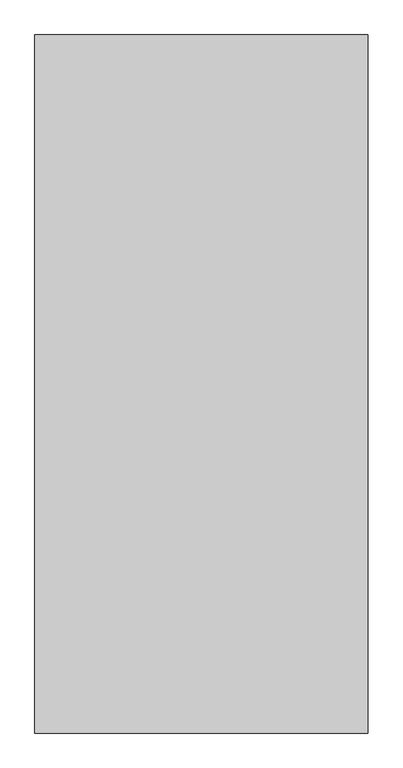
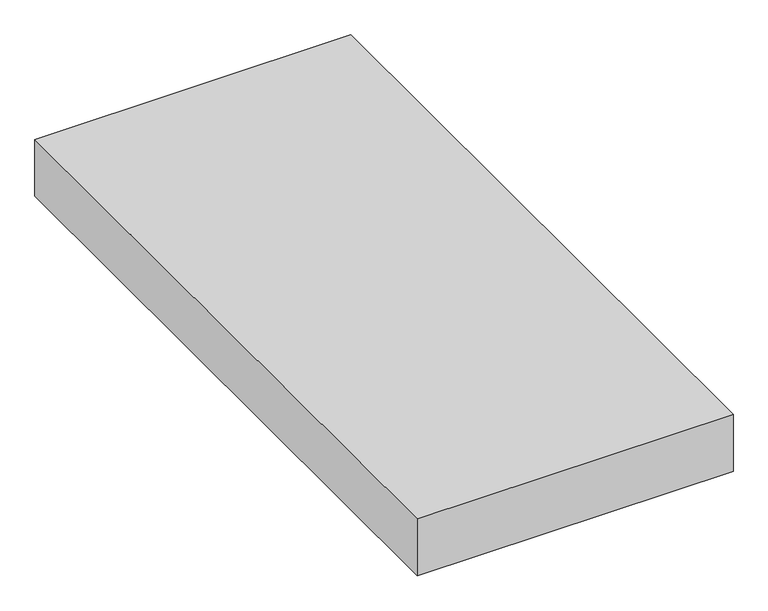
"""IFC4 building model written with IfcOpenShell, lengths in millimetres: proxy geometry, Space Planning Box_hec : Space Planning Box_hec."""

import ifcopenshell
import ifcopenshell.guid

model = None  # the IFC model being written
_history = None  # IfcOwnerHistory: only IFC2X3 demands one
_inside = {}  # id of a spatial element -> (the spatial element, [elements in it])
_under = {}  # id of a project, library or spatial element -> (it, [spatial elements below it])
_declared = {}  # id of a project -> (the project, [libraries it declares])
_typed = {}  # id of a type object -> (the type object, [elements of that type])
_made_of = {}  # id of a material, layer set ... -> (it, [elements and type objects made of it])


def new_model(schema):
    """Start an empty IFC model of exactly this schema.

    Asked for "IFC4X3", IfcOpenShell would pick the latest addendum, in which some entities
    have other attributes; the version numbers below select the first issue.
    IFC2X3 requires an IfcOwnerHistory on every rooted entity: one is made here for all.
    """
    global model, _history
    if schema == "IFC4X3":
        model = ifcopenshell.file(schema_version=(4, 3, 0, 0))
    else:
        model = ifcopenshell.file(schema=schema)
    _inside.clear()
    _under.clear()
    _declared.clear()
    _typed.clear()
    _made_of.clear()
    _history = None
    if model.schema == "IFC2X3":
        org = make("IfcOrganization", Name="unknown")
        user = make(
            "IfcPersonAndOrganization",
            ThePerson=make("IfcPerson", FamilyName="unknown"),
            TheOrganization=org,
        )
        app = make(
            "IfcApplication",
            ApplicationDeveloper=org,
            Version="unknown",
            ApplicationFullName="unknown",
            ApplicationIdentifier="unknown",
        )
        _history = make(
            "IfcOwnerHistory",
            OwningUser=user,
            OwningApplication=app,
            ChangeAction="ADDED",
            CreationDate=0,
        )
    return model


def make(cls, **values):
    """One entity of the class cls with the attributes given. An attribute that is None is left unset."""
    return model.create_entity(
        cls, **{name: value for name, value in values.items() if value is not None}
    )


def rooted(cls, **values):
    """An entity with a GlobalId (a new one), such as an element, a storey or a relation."""
    return make(cls, GlobalId=ifcopenshell.guid.new(), OwnerHistory=_history, **values)


def si_unit(unit_type, name, prefix=None):
    """IfcSIUnit, for example si_unit("LENGTHUNIT", "METRE", prefix="MILLI")."""
    return make("IfcSIUnit", UnitType=unit_type, Prefix=prefix, Name=name)


def assignment(units):
    """IfcUnitAssignment: the units of a project."""
    return None if units is None else make("IfcUnitAssignment", Units=units)


def point(xyz):
    """IfcCartesianPoint."""
    return None if xyz is None else make("IfcCartesianPoint", Coordinates=xyz)


def direction(xyz):
    """IfcDirection."""
    return None if xyz is None else make("IfcDirection", DirectionRatios=xyz)


def frame(location, z_axis=None, x_axis=None):
    """IfcAxis2Placement3D, a coordinate frame: its origin and axes. An axis left out is left unset."""
    return make(
        "IfcAxis2Placement3D",
        Location=point(location),
        Axis=direction(z_axis),
        RefDirection=direction(x_axis),
    )


def origin():
    """The frame at (0, 0, 0) with its axes left unset."""
    return frame((0.0, 0.0, 0.0))


def origin_with_axes():
    """The frame at (0, 0, 0) with the z axis (0, 0, 1) and the x axis (1, 0, 0) written out."""
    return frame((0.0, 0.0, 0.0), z_axis=(0.0, 0.0, 1.0), x_axis=(1.0, 0.0, 0.0))


def place(relative_to, where):
    """IfcLocalPlacement: puts the frame where relative to a parent placement (None: the world)."""
    return make(
        "IfcLocalPlacement", PlacementRelTo=relative_to, RelativePlacement=where
    )


def context(
    kind, dimensions, precision=None, world=None, true_north=None, identifier=None
):
    """IfcGeometricRepresentationContext, for example the 3D "Model" context."""
    return make(
        "IfcGeometricRepresentationContext",
        ContextIdentifier=identifier,
        ContextType=kind,
        CoordinateSpaceDimension=dimensions,
        Precision=precision,
        WorldCoordinateSystem=world,
        TrueNorth=true_north,
    )


def project(units=None, contexts=None):
    """IfcProject with its units and contexts."""
    return rooted(
        "IfcProject",
        Name="project",
        RepresentationContexts=contexts,
        UnitsInContext=assignment(units),
    )


def spatial(cls, under=None, at=None, **own):
    """A site, building, storey or space (cls), placed at a placement, below another one or the project."""
    s = rooted(cls, ObjectPlacement=at, **own)
    if under is not None:
        _under.setdefault(under.id(), (under, []))[1].append(s)
    return s


def polyline(points):
    """IfcPolyline through the points."""
    return make("IfcPolyline", Points=[point(p) for p in points])


def outline(outer, holes=None, kind="AREA"):
    """IfcArbitraryClosedProfileDef: a profile drawn as a closed curve; with holes, ...WithVoids."""
    if holes is None:
        return make("IfcArbitraryClosedProfileDef", ProfileType=kind, OuterCurve=outer)
    return make(
        "IfcArbitraryProfileDefWithVoids",
        ProfileType=kind,
        OuterCurve=outer,
        InnerCurves=holes,
    )


def extrude(swept, where, along, depth):
    """IfcExtrudedAreaSolid: the profile swept, set in the frame where, extruded along a direction by depth."""
    return make(
        "IfcExtrudedAreaSolid",
        SweptArea=swept,
        Position=where,
        ExtrudedDirection=direction(along),
        Depth=depth,
    )


def shape(context_of_items, identifier, shape_type, items):
    """IfcShapeRepresentation: the items that make up one representation, for example the "Body"."""
    return make(
        "IfcShapeRepresentation",
        ContextOfItems=context_of_items,
        RepresentationIdentifier=identifier,
        RepresentationType=shape_type,
        Items=items,
    )


def source(mapping_origin, context_of_items, identifier, shape_type, items):
    """IfcRepresentationMap: a shape defined once, which mapped items show again and again."""
    return make(
        "IfcRepresentationMap",
        MappingOrigin=mapping_origin,
        MappedRepresentation=shape(context_of_items, identifier, shape_type, items),
    )


def transform(
    local_origin,
    x_axis=None,
    y_axis=None,
    z_axis=None,
    scale=None,
    scale2=None,
    scale3=None,
    uniform=True,
):
    """IfcCartesianTransformationOperator3D, or its non-uniform kind. x_axis, y_axis, z_axis: its Axis1, 2, 3."""
    if uniform:
        return make(
            "IfcCartesianTransformationOperator3D",
            Axis1=direction(x_axis),
            Axis2=direction(y_axis),
            LocalOrigin=point(local_origin),
            Scale=scale,
            Axis3=direction(z_axis),
        )
    return make(
        "IfcCartesianTransformationOperator3DnonUniform",
        Axis1=direction(x_axis),
        Axis2=direction(y_axis),
        LocalOrigin=point(local_origin),
        Scale=scale,
        Axis3=direction(z_axis),
        Scale2=scale2,
        Scale3=scale3,
    )


def mapped(mapping_source, mapping_target):
    """IfcMappedItem: shows the shape of a source again, moved by a transform."""
    return make(
        "IfcMappedItem", MappingSource=mapping_source, MappingTarget=mapping_target
    )


def made_of(thing, what):
    """Note that an element or type object is made of a material, layer set ...; save() writes the relation."""
    if what is not None:
        _made_of.setdefault(what.id(), (what, []))[1].append(thing)
    return thing


def element(
    cls,
    number,
    at=None,
    inside=None,
    cuts=None,
    type_object=None,
    material=None,
    context=None,
    identifier="Body",
    shape_type=None,
    held_by="IfcProductDefinitionShape",
    body=None,
    shapes=None,
    **own,
):
    """One element of the class cls, such as IfcWall. Its Tag is "e" and its number.

    at: its placement. inside: the storey or other place that contains it. cuts: it is an
    opening in that element (IfcRelVoidsElement). A single representation is given by context,
    identifier, shape_type and body (its items); several are given by shapes. held_by: the class
    of the entity that holds the representations. save() writes the other relations.
    """
    e = rooted(cls, Tag="e%d" % number, ObjectPlacement=at, **own)
    if body is not None:
        shapes = [shape(context, identifier, shape_type, body)]
    if shapes is not None:
        e.Representation = make(held_by, Representations=shapes)
    if inside is not None:
        _inside.setdefault(inside.id(), (inside, []))[1].append(e)
    if cuts is not None:
        rooted(
            "IfcRelVoidsElement", RelatingBuildingElement=cuts, RelatedOpeningElement=e
        )
    if type_object is not None:
        _typed.setdefault(type_object.id(), (type_object, []))[1].append(e)
    return made_of(e, material)


def aggregate(whole, parts):
    """IfcRelAggregates: a whole, such as a stair, and the parts it consists of."""
    return rooted("IfcRelAggregates", RelatingObject=whole, RelatedObjects=parts)


def save(model, path):
    """Write the relations noted so far, then the file.

    IfcRelAggregates (storeys below a building ...), IfcRelContainedInSpatialStructure (elements
    in a storey), IfcRelDefinesByType, IfcRelAssociatesMaterial and IfcRelDeclares: one each for
    every whole, place, type object, material and project.
    """
    for whole, parts in _under.values():
        aggregate(whole, parts)
    for where, things in _inside.values():
        rooted(
            "IfcRelContainedInSpatialStructure",
            RelatedElements=things,
            RelatingStructure=where,
        )
    for kind, things in _typed.values():
        rooted("IfcRelDefinesByType", RelatedObjects=things, RelatingType=kind)
    for what, things in _made_of.values():
        rooted("IfcRelAssociatesMaterial", RelatedObjects=things, RelatingMaterial=what)
    for by, libraries in _declared.values():
        rooted("IfcRelDeclares", RelatingContext=by, RelatedDefinitions=libraries)
    model.write(path)


def generic_models_a454a2aa(model_context):
    return source(origin(), model_context, "Body", "SweptSolid", [
        extrude(outline(polyline([(10500.0, 22000.0), (10500.0, -22000.0), (-10500.0, -22000.0), (-10500.0, 22000.0), (10500.0, 22000.0)])), origin_with_axes(), (0.0, 0.0, 1.0), 4000.0),
    ])


if __name__ == "__main__":
    model = new_model("IFC4")
    model_context = context("Model", 3, world=origin())
    ifc_project = project(units=[si_unit("LENGTHUNIT", "METRE", prefix="MILLI")], contexts=[model_context])
    site = spatial("IfcSite", under=ifc_project)
    building = spatial("IfcBuilding", under=site)
    placement = place(None, origin())
    generic_models_shape = generic_models_a454a2aa(model_context)
    element("IfcBuildingElementProxy", 1, Name="Space Planning Box_hec : Space Planning Box_hec", ObjectType="Space Planning Box_hec : Space Planning Box_hec", at=placement, inside=building, context=model_context, shape_type="MappedRepresentation", body=[
        mapped(generic_models_shape, transform((0.0, 0.0, 0.0), x_axis=(1.0, 0.0, 0.0), y_axis=(0.0, 1.0, 0.0), z_axis=(0.0, 0.0, 1.0))),
    ])
    save(model, "model.ifc")

# Revit data of these elements
# Type "Space Planning Box_hec : Space Planning Box_hec"
#   Type Comments = "..."
#   Room Name [instance default] = "?"
#   Interior Finish [instance default] = ""
#   Exterior Finish [instance default] = ""
#   Department [instance default] = ""
#   Assembly Code = "..."
#   Width [instance default] = 1524 mm
#   Program Area [instance default] = 0.00 m²
#   Length [instance default] = 1524 mm
#   Height [instance default] = 1524 mm
#   Area [instance default] = 2.32258 m²
#   Fill Color [instance default] = Cyan
#   Default Elevation = 0
# Element 1 (IfcBuildingElementProxy, "Space Planning Box_hec : Space Planning Box_hec")
#   Room Name = "Cable Room"
#   Interior Finish = "IF1"
#   Exterior Finish = "EF1"
#   Department = "EL"
#   Width = 21000 mm
#   Program Area = 924.00 m²
#   Length = 44000 mm
#   Height = 4000 mm
#   Area = 924.00 m²
#   Fill Color = Blue
#   Materials on its faces: "Blue"
# Materials
#   "Cyan": class "Generic", colour RGB 0 255 255, transparency 0.2, Cost = 0
#   "Blue": class "Generic", colour RGB 0 0 255, transparency 0.2, Cost = 0
